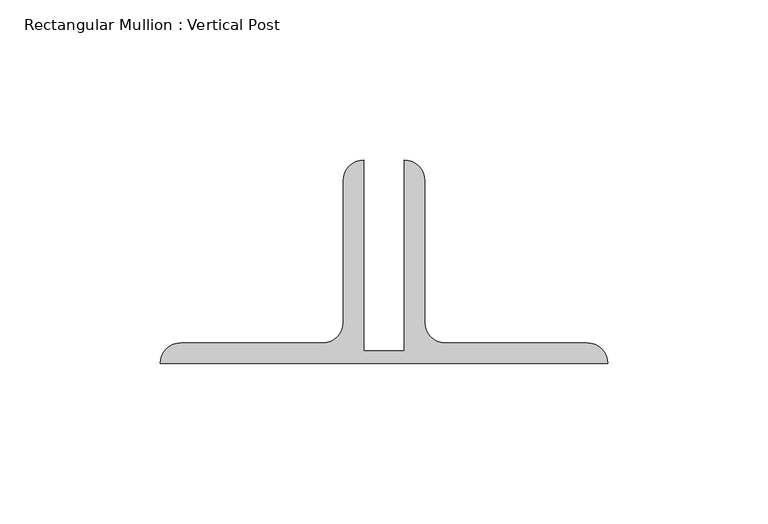
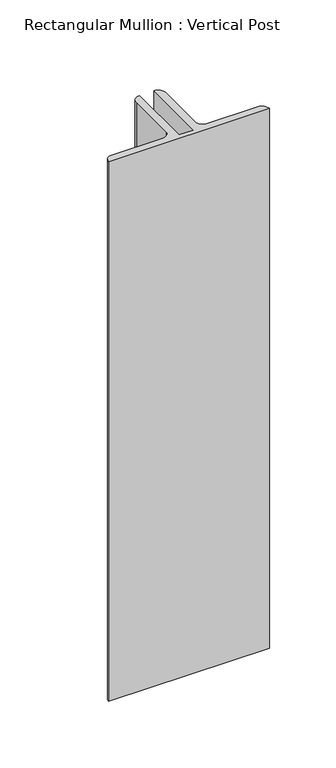
"""IFC4 building model written with IfcOpenShell, lengths in millimetres: member geometry, Rectangular Mullion : Vertical Post."""

from ifc_helpers import new_model, si_unit, point, frame, frame_2d, origin, place, context, project, spatial, polyline, circle_curve, trimmed, segment, composite_curve, outline, extrude, source, transform, mapped, element, save


def rectangular_mullion_vertical_post_4e0e3b0c(model_context):
    return source(origin(), model_context, "Body", "SweptSolid", [
        extrude(outline(composite_curve([segment(polyline([(-63.5, 22.9145205), (-63.5, 82.55)]), True, "CONTINUOUS"), segment(trimmed(circle_curve(frame_2d((-63.5, 76.2)), 6.35), [point((-63.5, 82.55))], [point((-57.15, 76.2))], False, "CARTESIAN"), True, "CONTINUOUS"), segment(polyline([(-57.15, 76.2), (-57.15, 31.75)]), True, "CONTINUOUS"), segment(trimmed(circle_curve(frame_2d((-50.8, 31.75)), 6.35), [point((-57.15, 31.75))], [point((-50.8, 25.4))], True, "CARTESIAN"), True, "CONTINUOUS"), segment(polyline([(-50.8, 25.4), (-6.35, 25.4)]), True, "CONTINUOUS"), segment(trimmed(circle_curve(frame_2d((-6.35, 19.05)), 6.35), [point((-6.35, 25.4))], [point((0.0, 19.05))], False, "CARTESIAN"), True, "CONTINUOUS"), segment(polyline([(0.0, 19.05), (-139.7, 19.05)]), True, "CONTINUOUS"), segment(trimmed(circle_curve(frame_2d((-133.35, 19.05)), 6.35), [point((-139.7, 19.05))], [point((-133.35, 25.4))], False, "CARTESIAN"), True, "CONTINUOUS"), segment(polyline([(-133.35, 25.4), (-88.9, 25.4)]), True, "CONTINUOUS"), segment(trimmed(circle_curve(frame_2d((-88.9, 31.75)), 6.35), [point((-88.9, 25.4))], [point((-82.55, 31.75))], True, "CARTESIAN"), True, "CONTINUOUS"), segment(polyline([(-82.55, 31.75), (-82.55, 76.2)]), True, "CONTINUOUS"), segment(trimmed(circle_curve(frame_2d((-76.2, 76.2)), 6.35), [point((-82.55, 76.2))], [point((-76.2, 82.55))], False, "CARTESIAN"), True, "CONTINUOUS"), segment(polyline([(-76.2, 82.55), (-76.2, 22.9145205), (-63.5, 22.9145205)]), True, "CONTINUOUS")], self_intersect=False)), frame((0.0, 0.0, -495.3992188), z_axis=(0.0, 0.0, 1.0), x_axis=(1.0, 0.0, 0.0)), (0.0, 0.0, 1.0), 495.3992188),
    ])


if __name__ == "__main__":
    model = new_model("IFC4")
    model_context = context("Model", 3, world=origin())
    ifc_project = project(units=[si_unit("LENGTHUNIT", "METRE", prefix="MILLI")], contexts=[model_context])
    site = spatial("IfcSite", under=ifc_project)
    building = spatial("IfcBuilding", under=site)
    placement = place(None, origin())
    rectangular_mullion_vertical_post_shape = rectangular_mullion_vertical_post_4e0e3b0c(model_context)
    element("IfcMember", 1, ObjectType="Rectangular Mullion : Vertical Post", at=placement, inside=building, context=model_context, shape_type="MappedRepresentation", body=[
        mapped(rectangular_mullion_vertical_post_shape, transform((0.0, 0.0, 0.0), x_axis=(1.0, 0.0, 0.0), y_axis=(0.0, 1.0, 0.0), z_axis=(0.0, 0.0, 1.0))),
    ])
    save(model, "model.ifc")

# Revit data of these elements
# Type "Rectangular Mullion : Vertical Post"
#   built-in parameter 1007351 = -0.0625 (stored number, unit not read)
#   built-in parameter 1007322 = 0.0126789 (stored number, unit not read)
#   built-in parameter 1007321 = 0.229167 (stored number, unit not read)
#   built-in parameter 1007320 = 0.229167 (stored number, unit not read)
# Element 1 (IfcMember, "Rectangular Mullion : Vertical Post")
#   Materials on its faces: "GATE POST: (2) BACK/BACK GALVANIZED ANGLES"
# Materials
#   "GATE POST: (2) BACK/BACK GALVANIZED ANGLES": class "Unassigned", colour RGB 211 211 211, transparency 0, Cost = 0
